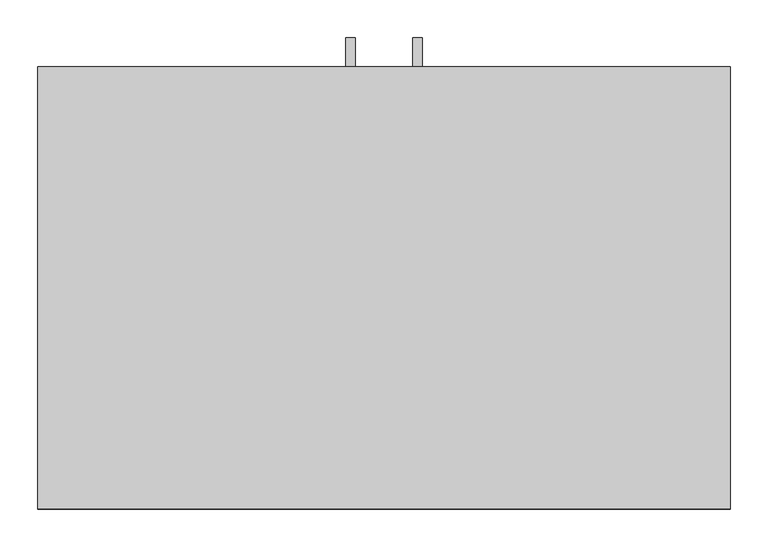
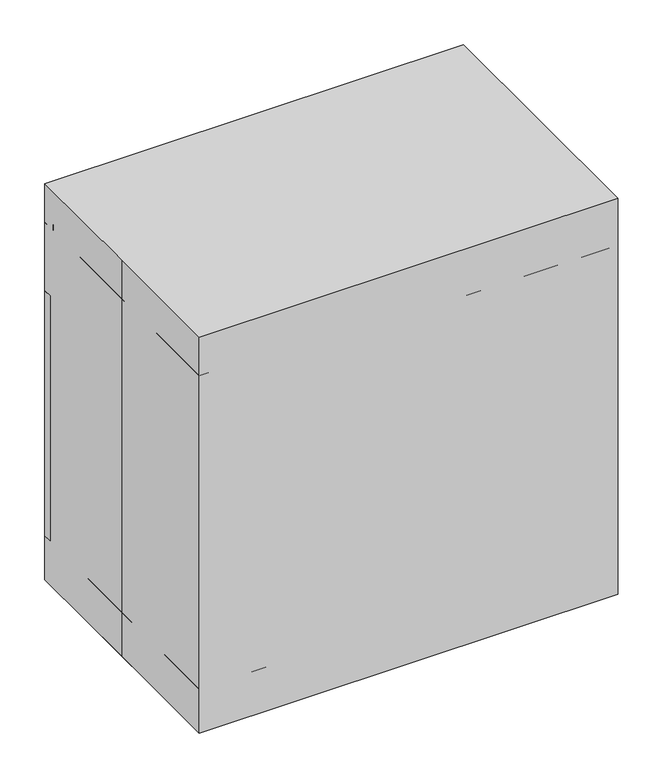
"""IFC4 building model written with IfcOpenShell, lengths in millimetres: proxy geometry, C04P0 - Cabinet, Sink, U-C-B, 2 Door, 36x36x22 : C04P0 - Cabinet, Sink, U-C-B, 2 Door, 36x36x22."""

import ifcopenshell
import ifcopenshell.guid

model = None  # the IFC model being written
_history = None  # IfcOwnerHistory: only IFC2X3 demands one
_inside = {}  # id of a spatial element -> (the spatial element, [elements in it])
_under = {}  # id of a project, library or spatial element -> (it, [spatial elements below it])
_declared = {}  # id of a project -> (the project, [libraries it declares])
_typed = {}  # id of a type object -> (the type object, [elements of that type])
_made_of = {}  # id of a material, layer set ... -> (it, [elements and type objects made of it])


def new_model(schema):
    """Start an empty IFC model of exactly this schema.

    Asked for "IFC4X3", IfcOpenShell would pick the latest addendum, in which some entities
    have other attributes; the version numbers below select the first issue.
    IFC2X3 requires an IfcOwnerHistory on every rooted entity: one is made here for all.
    """
    global model, _history
    if schema == "IFC4X3":
        model = ifcopenshell.file(schema_version=(4, 3, 0, 0))
    else:
        model = ifcopenshell.file(schema=schema)
    _inside.clear()
    _under.clear()
    _declared.clear()
    _typed.clear()
    _made_of.clear()
    _history = None
    if model.schema == "IFC2X3":
        org = make("IfcOrganization", Name="unknown")
        user = make(
            "IfcPersonAndOrganization",
            ThePerson=make("IfcPerson", FamilyName="unknown"),
            TheOrganization=org,
        )
        app = make(
            "IfcApplication",
            ApplicationDeveloper=org,
            Version="unknown",
            ApplicationFullName="unknown",
            ApplicationIdentifier="unknown",
        )
        _history = make(
            "IfcOwnerHistory",
            OwningUser=user,
            OwningApplication=app,
            ChangeAction="ADDED",
            CreationDate=0,
        )
    return model


def make(cls, **values):
    """One entity of the class cls with the attributes given. An attribute that is None is left unset."""
    return model.create_entity(
        cls, **{name: value for name, value in values.items() if value is not None}
    )


def rooted(cls, **values):
    """An entity with a GlobalId (a new one), such as an element, a storey or a relation."""
    return make(cls, GlobalId=ifcopenshell.guid.new(), OwnerHistory=_history, **values)


def si_unit(unit_type, name, prefix=None):
    """IfcSIUnit, for example si_unit("LENGTHUNIT", "METRE", prefix="MILLI")."""
    return make("IfcSIUnit", UnitType=unit_type, Prefix=prefix, Name=name)


def assignment(units):
    """IfcUnitAssignment: the units of a project."""
    return None if units is None else make("IfcUnitAssignment", Units=units)


def point(xyz):
    """IfcCartesianPoint."""
    return None if xyz is None else make("IfcCartesianPoint", Coordinates=xyz)


def direction(xyz):
    """IfcDirection."""
    return None if xyz is None else make("IfcDirection", DirectionRatios=xyz)


def frame(location, z_axis=None, x_axis=None):
    """IfcAxis2Placement3D, a coordinate frame: its origin and axes. An axis left out is left unset."""
    return make(
        "IfcAxis2Placement3D",
        Location=point(location),
        Axis=direction(z_axis),
        RefDirection=direction(x_axis),
    )


def origin():
    """The frame at (0, 0, 0) with its axes left unset."""
    return frame((0.0, 0.0, 0.0))


def origin_with_axes():
    """The frame at (0, 0, 0) with the z axis (0, 0, 1) and the x axis (1, 0, 0) written out."""
    return frame((0.0, 0.0, 0.0), z_axis=(0.0, 0.0, 1.0), x_axis=(1.0, 0.0, 0.0))


def place(relative_to, where):
    """IfcLocalPlacement: puts the frame where relative to a parent placement (None: the world)."""
    return make(
        "IfcLocalPlacement", PlacementRelTo=relative_to, RelativePlacement=where
    )


def context(
    kind, dimensions, precision=None, world=None, true_north=None, identifier=None
):
    """IfcGeometricRepresentationContext, for example the 3D "Model" context."""
    return make(
        "IfcGeometricRepresentationContext",
        ContextIdentifier=identifier,
        ContextType=kind,
        CoordinateSpaceDimension=dimensions,
        Precision=precision,
        WorldCoordinateSystem=world,
        TrueNorth=true_north,
    )


def project(units=None, contexts=None):
    """IfcProject with its units and contexts."""
    return rooted(
        "IfcProject",
        Name="project",
        RepresentationContexts=contexts,
        UnitsInContext=assignment(units),
    )


def spatial(cls, under=None, at=None, **own):
    """A site, building, storey or space (cls), placed at a placement, below another one or the project."""
    s = rooted(cls, ObjectPlacement=at, **own)
    if under is not None:
        _under.setdefault(under.id(), (under, []))[1].append(s)
    return s


def polyline(points):
    """IfcPolyline through the points."""
    return make("IfcPolyline", Points=[point(p) for p in points])


def outline(outer, holes=None, kind="AREA"):
    """IfcArbitraryClosedProfileDef: a profile drawn as a closed curve; with holes, ...WithVoids."""
    if holes is None:
        return make("IfcArbitraryClosedProfileDef", ProfileType=kind, OuterCurve=outer)
    return make(
        "IfcArbitraryProfileDefWithVoids",
        ProfileType=kind,
        OuterCurve=outer,
        InnerCurves=holes,
    )


def extrude(swept, where, along, depth):
    """IfcExtrudedAreaSolid: the profile swept, set in the frame where, extruded along a direction by depth."""
    return make(
        "IfcExtrudedAreaSolid",
        SweptArea=swept,
        Position=where,
        ExtrudedDirection=direction(along),
        Depth=depth,
    )


def shape(context_of_items, identifier, shape_type, items):
    """IfcShapeRepresentation: the items that make up one representation, for example the "Body"."""
    return make(
        "IfcShapeRepresentation",
        ContextOfItems=context_of_items,
        RepresentationIdentifier=identifier,
        RepresentationType=shape_type,
        Items=items,
    )


def source(mapping_origin, context_of_items, identifier, shape_type, items):
    """IfcRepresentationMap: a shape defined once, which mapped items show again and again."""
    return make(
        "IfcRepresentationMap",
        MappingOrigin=mapping_origin,
        MappedRepresentation=shape(context_of_items, identifier, shape_type, items),
    )


def transform(
    local_origin,
    x_axis=None,
    y_axis=None,
    z_axis=None,
    scale=None,
    scale2=None,
    scale3=None,
    uniform=True,
):
    """IfcCartesianTransformationOperator3D, or its non-uniform kind. x_axis, y_axis, z_axis: its Axis1, 2, 3."""
    if uniform:
        return make(
            "IfcCartesianTransformationOperator3D",
            Axis1=direction(x_axis),
            Axis2=direction(y_axis),
            LocalOrigin=point(local_origin),
            Scale=scale,
            Axis3=direction(z_axis),
        )
    return make(
        "IfcCartesianTransformationOperator3DnonUniform",
        Axis1=direction(x_axis),
        Axis2=direction(y_axis),
        LocalOrigin=point(local_origin),
        Scale=scale,
        Axis3=direction(z_axis),
        Scale2=scale2,
        Scale3=scale3,
    )


def mapped(mapping_source, mapping_target):
    """IfcMappedItem: shows the shape of a source again, moved by a transform."""
    return make(
        "IfcMappedItem", MappingSource=mapping_source, MappingTarget=mapping_target
    )


def made_of(thing, what):
    """Note that an element or type object is made of a material, layer set ...; save() writes the relation."""
    if what is not None:
        _made_of.setdefault(what.id(), (what, []))[1].append(thing)
    return thing


def element(
    cls,
    number,
    at=None,
    inside=None,
    cuts=None,
    type_object=None,
    material=None,
    context=None,
    identifier="Body",
    shape_type=None,
    held_by="IfcProductDefinitionShape",
    body=None,
    shapes=None,
    **own,
):
    """One element of the class cls, such as IfcWall. Its Tag is "e" and its number.

    at: its placement. inside: the storey or other place that contains it. cuts: it is an
    opening in that element (IfcRelVoidsElement). A single representation is given by context,
    identifier, shape_type and body (its items); several are given by shapes. held_by: the class
    of the entity that holds the representations. save() writes the other relations.
    """
    e = rooted(cls, Tag="e%d" % number, ObjectPlacement=at, **own)
    if body is not None:
        shapes = [shape(context, identifier, shape_type, body)]
    if shapes is not None:
        e.Representation = make(held_by, Representations=shapes)
    if inside is not None:
        _inside.setdefault(inside.id(), (inside, []))[1].append(e)
    if cuts is not None:
        rooted(
            "IfcRelVoidsElement", RelatingBuildingElement=cuts, RelatedOpeningElement=e
        )
    if type_object is not None:
        _typed.setdefault(type_object.id(), (type_object, []))[1].append(e)
    return made_of(e, material)


def aggregate(whole, parts):
    """IfcRelAggregates: a whole, such as a stair, and the parts it consists of."""
    return rooted("IfcRelAggregates", RelatingObject=whole, RelatedObjects=parts)


def save(model, path):
    """Write the relations noted so far, then the file.

    IfcRelAggregates (storeys below a building ...), IfcRelContainedInSpatialStructure (elements
    in a storey), IfcRelDefinesByType, IfcRelAssociatesMaterial and IfcRelDeclares: one each for
    every whole, place, type object, material and project.
    """
    for whole, parts in _under.values():
        aggregate(whole, parts)
    for where, things in _inside.values():
        rooted(
            "IfcRelContainedInSpatialStructure",
            RelatedElements=things,
            RelatingStructure=where,
        )
    for kind, things in _typed.values():
        rooted("IfcRelDefinesByType", RelatedObjects=things, RelatingType=kind)
    for what, things in _made_of.values():
        rooted("IfcRelAssociatesMaterial", RelatedObjects=things, RelatingMaterial=what)
    for by, libraries in _declared.values():
        rooted("IfcRelDeclares", RelatingContext=by, RelatedDefinitions=libraries)
    model.write(path)


def specialty_equipment_691782c5(model_context):
    return source(origin(), model_context, "Body", "SweptSolid", [
        extrude(outline(polyline([(330.2, 518.5968273), (292.1, 518.5968273), (292.1, 531.2808974), (317.5159299, 531.2808974), (317.5159299, 601.1627573), (292.1, 601.1627573), (292.1, 613.8468273), (330.2, 613.8468273), (330.2, 518.5968273)])), frame((38.1, 0.0, 0.0), z_axis=(1.0, 0.0, 0.0), x_axis=(0.0, 1.0, 0.0)), (0.0, 0.0, 1.0), 12.7),
        extrude(outline(polyline([(330.2, 518.5968273), (292.1, 518.5968273), (292.1, 531.2808974), (317.5159299, 531.2808974), (317.5159299, 601.1627573), (292.1, 601.1627573), (292.1, 613.8468273), (330.2, 613.8468273), (330.2, 518.5968273)])), frame((-50.8, 0.0, 0.0), z_axis=(1.0, 0.0, 0.0), x_axis=(0.0, 1.0, 0.0)), (0.0, 0.0, 1.0), 12.7),
        extrude(outline(polyline([(0.0, 292.1), (0.0, 273.05), (-457.2, 273.05), (-457.2, 292.1), (0.0, 292.1)])), frame((0.0, 0.0, 101.6), z_axis=(0.0, 0.0, 1.0), x_axis=(1.0, 0.0, 0.0)), (0.0, 0.0, 1.0), 565.15),
        extrude(outline(polyline([(457.2, 292.1), (457.2, 273.05), (0.0, 273.05), (0.0, 292.1), (457.2, 292.1)])), frame((0.0, 0.0, 101.6), z_axis=(0.0, 0.0, 1.0), x_axis=(1.0, 0.0, 0.0)), (0.0, 0.0, 1.0), 565.15),
        extrude(outline(polyline([(-457.2, -292.1), (-457.2, 0.0), (-457.2, 292.1), (457.2, 292.1), (457.2, -292.1), (-457.2, -292.1)])), origin_with_axes(), (0.0, 0.0, 1.0), 914.4),
        extrude(outline(polyline([(438.15, 260.35), (-438.15, 260.35), (-438.15, 273.05), (438.15, 273.05), (438.15, 260.35)])), frame((0.0, 0.0, 641.0750636), z_axis=(0.0, 0.0, 1.0), x_axis=(1.0, 0.0, 0.0)), (0.0, 0.0, 1.0), 51.0749364),
        extrude(outline(polyline([(457.2, 292.1), (457.2, 273.05), (-457.2, 273.05), (-457.2, 292.1), (457.2, 292.1)])), frame((0.0, 0.0, 673.1), z_axis=(0.0, 0.0, 1.0), x_axis=(1.0, 0.0, 0.0)), (0.0, 0.0, 1.0), 152.4),
        extrude(outline(polyline([(-457.2, 273.05), (-438.15, 273.05), (-438.15, -292.1), (-457.2, -292.1), (-457.2, 273.05)])), frame((0.0, 0.0, 101.6), z_axis=(0.0, 0.0, 1.0), x_axis=(1.0, 0.0, 0.0)), (0.0, 0.0, 1.0), 723.9),
        extrude(outline(polyline([(438.15, 273.05), (457.2, 273.05), (457.2, -292.1), (438.15, -292.1), (438.15, 273.05)])), frame((0.0, 0.0, 101.6), z_axis=(0.0, 0.0, 1.0), x_axis=(1.0, 0.0, 0.0)), (0.0, 0.0, 1.0), 723.9),
        extrude(outline(polyline([(457.2, 260.35), (-457.2, 260.35), (-457.2, 273.05), (457.2, 273.05), (457.2, 260.35)])), frame((0.0, 0.0, 825.5), z_axis=(0.0, 0.0, 1.0), x_axis=(1.0, 0.0, 0.0)), (0.0, 0.0, 1.0), 12.7),
        extrude(outline(polyline([(457.2, 234.95), (457.2, 215.9), (-457.2, 215.9), (-457.2, 234.95), (457.2, 234.95)])), origin_with_axes(), (0.0, 0.0, 1.0), 101.6),
        extrude(outline(polyline([(-457.2, 215.9), (-438.15, 215.9), (-438.15, -292.1), (-457.2, -292.1), (-457.2, 215.9)])), origin_with_axes(), (0.0, 0.0, 1.0), 101.6),
        extrude(outline(polyline([(438.15, 215.9), (457.2, 215.9), (457.2, -285.75), (438.15, -285.75), (438.15, 215.9)])), origin_with_axes(), (0.0, 0.0, 1.0), 101.6),
        extrude(outline(polyline([(457.2, -273.05), (457.2, -292.1), (-457.2, -292.1), (-457.2, -273.05), (457.2, -273.05)])), origin_with_axes(), (0.0, 0.0, 1.0), 101.6),
        extrude(outline(polyline([(438.15, -273.05), (-438.15, -273.05), (-438.15, 273.05), (438.15, 273.05), (438.15, -273.05)])), frame((0.0, 0.0, 101.6), z_axis=(0.0, 0.0, 1.0), x_axis=(1.0, 0.0, 0.0)), (0.0, 0.0, 1.0), 19.1166954),
        extrude(outline(polyline([(438.15, -273.05), (438.15, -292.1), (-438.15, -292.1), (-438.15, -273.05), (438.15, -273.05)])), frame((0.0, 0.0, 101.6), z_axis=(0.0, 0.0, 1.0), x_axis=(1.0, 0.0, 0.0)), (0.0, 0.0, 1.0), 704.85),
    ])


if __name__ == "__main__":
    model = new_model("IFC4")
    model_context = context("Model", 3, world=origin())
    ifc_project = project(units=[si_unit("LENGTHUNIT", "METRE", prefix="MILLI")], contexts=[model_context])
    site = spatial("IfcSite", under=ifc_project)
    building = spatial("IfcBuilding", under=site)
    placement = place(None, origin())
    specialty_equipment_shape = specialty_equipment_691782c5(model_context)
    element("IfcBuildingElementProxy", 1, Name="C04P0 - Cabinet, Sink, U-C-B, 2 Door, 36x36x22 : C04P0 - Cabinet, Sink, U-C-B, 2 Door, 36x36x22", ObjectType="C04P0 - Cabinet, Sink, U-C-B, 2 Door, 36x36x22 : C04P0 - Cabinet, Sink, U-C-B, 2 Door, 36x36x22", at=placement, inside=building, context=model_context, shape_type="MappedRepresentation", body=[
        mapped(specialty_equipment_shape, transform((0.0, 0.0, 0.0), x_axis=(1.0, 0.0, 0.0), y_axis=(0.0, 1.0, 0.0), z_axis=(0.0, 0.0, 1.0))),
    ])
    save(model, "model.ifc")

# Revit data of these elements
# Type "C04P0 - Cabinet, Sink, U-C-B, 2 Door, 36x36x22 : C04P0 - Cabinet, Sink, U-C-B, 2 Door, 36x36x22"
#   Watts2 = "0"
#   Watts1 = "0"
#   Unit_Issue = "EA"
#   UTIL_6_Misc = "-"
#   UTIL_5_NonMedGas = "-"
#   UTIL_4_MiscGas = "-"
#   UTIL_3_MedGas = "-"
#   UTIL_2_Elec = "-"
#   UTIL_1_WaterDrain = "-"
#   Nomenclature = "Cabinet, Sink, U/C/B, 2 Door, 36x36x22"
#   NSN = "6530"
#   Location [instance default] = ""
#   JSN = "C04P0"
#   Fund_Source_VA = "-"
#   Fund_Source_Navy = "-"
#   Fund_Source_Army = "-"
#   Fund_Source_AF = "-"
#   ELEC_Volts2 = "0"
#   ELEC_Volts1 = "0"
#   ELEC_Phase2 = "0"
#   ELEC_Phase1 = "0"
#   ELEC_HertzSwitch = "0"
#   ELEC_HertzDependent = "0"
#   ELEC_Hertz = "0"
#   ELEC_Amps2 = "0"
#   ELEC_Amps1 = "0"
#   DetailDescription = "Standing height under counter base sink cabinet with solid hinged doors. Also referred to as a double-door sink cabinet. For general purpose use throughout the facility where a sink is to be used. Coordinate actual clear cabinet dimension with the actual outside dimension of sink that is specified to ensure that they are compatible."
#   CAT_VA = "A"
#   CAT_Navy = "A"
#   CAT_IHS = "-"
#   CAT_Army = "A"
#   CAT_AF = "A"
#   BTUperhour = "0"
#   Weight_IP = 115
#   DIM_Width_IP = 3' - 0"
#   DIM_Height_IP = 3' - 0"
#   DIM_Depth_IP = 1' - 11"
#   Shelf Panel Material = none
#   Assembly Code = ""
# Element 1 (IfcBuildingElementProxy, "C04P0 - Cabinet, Sink, U-C-B, 2 Door, 36x36x22 : C04P0 - Cabinet, Sink, U-C-B, 2 Door, 36x36x22")
#   Materials on its faces: "CabinetFinish", "Default metal", "EquipSpace"
# Materials
#   "CabinetFinish": class "Unassigned", colour RGB 245 239 218, transparency 0
#   "Default metal": class "Unassigned", colour RGB 204 204 204, transparency 0
#   "EquipSpace": class "Unassigned", colour RGB 221 217 195, transparency 0.5
